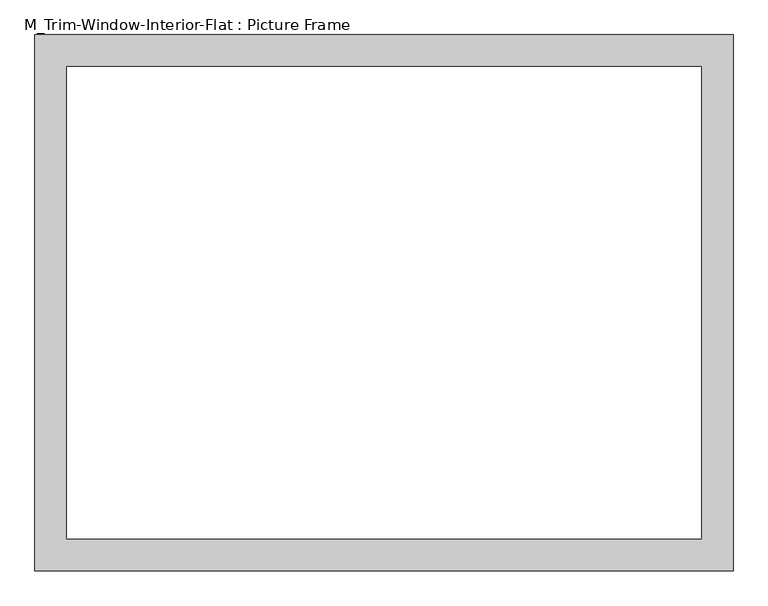
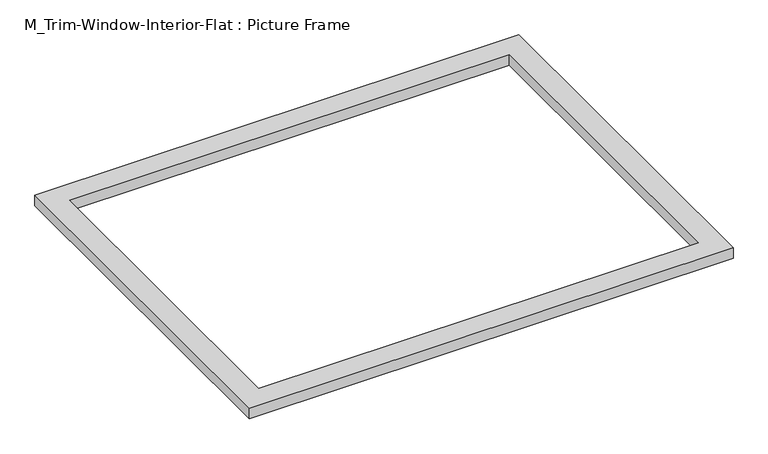
"""IFC4 building model written with IfcOpenShell, lengths in millimetres: proxy geometry, M_Trim-Window-Interior-Flat : Picture Frame."""

from ifc_helpers import new_model, si_unit, origin, origin_with_axes, place, context, project, spatial, polyline, outline, extrude, source, transform, mapped, element, save


def m_trim_window_interior_flat_picture_frame_c544af4f(model_context):
    return source(origin(), model_context, "Body", "SweptSolid", [
        extrude(outline(polyline([(656.9, -47.3), (-656.9, -47.3), (-656.9, 961.7), (656.9, 961.7), (656.9, -47.3)]), holes=[polyline([(596.9, 12.7), (596.9, 901.7), (-596.9, 901.7), (-596.9, 12.7), (596.9, 12.7)])]), origin_with_axes(), (0.0, 0.0, 1.0), 30.0),
    ])


if __name__ == "__main__":
    model = new_model("IFC4")
    model_context = context("Model", 3, world=origin())
    ifc_project = project(units=[si_unit("LENGTHUNIT", "METRE", prefix="MILLI")], contexts=[model_context])
    site = spatial("IfcSite", under=ifc_project)
    building = spatial("IfcBuilding", under=site)
    placement = place(None, origin())
    m_trim_window_interior_flat_picture_frame_shape = m_trim_window_interior_flat_picture_frame_c544af4f(model_context)
    element("IfcBuildingElementProxy", 1, Name="M_Trim-Window-Interior-Flat : Picture Frame", ObjectType="M_Trim-Window-Interior-Flat : Picture Frame", at=placement, inside=building, context=model_context, shape_type="MappedRepresentation", body=[
        mapped(m_trim_window_interior_flat_picture_frame_shape, transform((0.0, 0.0, 0.0), x_axis=(1.0, 0.0, 0.0), y_axis=(0.0, 1.0, 0.0), z_axis=(0.0, 0.0, 1.0))),
    ])
    save(model, "model.ifc")

# Revit data of these elements
# Type "M_Trim-Window-Interior-Flat : Picture Frame"
#   Trim Thickness_Picture Frame = 0' - 1.1811"
#   Trim Width = 0' - 2.3622"
#   Trim Thickness_with Sill = 0' - 0.7874"
#   Sill Thickness = 0' - 1.1811"
#   Opening Width [instance default] = 1' - 11.62205"
#   Opening Height [instance default] = 2' - 11.43307"
#   Default Elevation = 3' - 11.24409"
#   Sill = no
#   Picture Frame = yes
#   Trim Material [instance default] = none
# Element 1 (IfcBuildingElementProxy, "M_Trim-Window-Interior-Flat : Picture Frame")
#   Opening Width = 4' - 0"
#   Opening Height = 3' - 0"
#   Trim Material = Wood - Stained
#   Materials on its faces: "Wood - Stained"
# Materials
#   "Wood - Stained": class "Wood", colour RGB 224 178 126, transparency 0, Cost = 0
